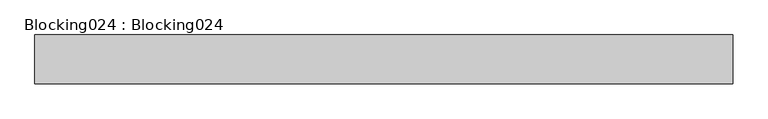
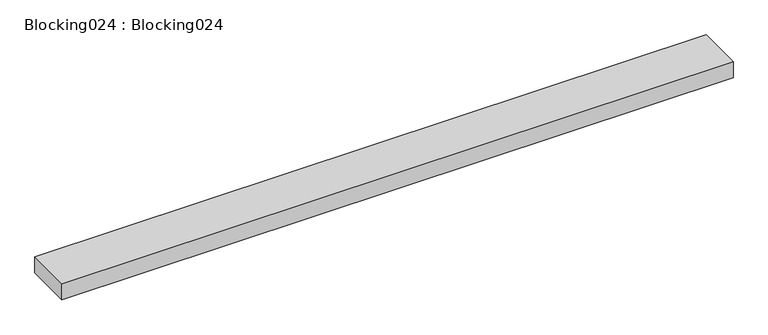
"""IFC4 building model written with IfcOpenShell, lengths in millimetres: proxy geometry, Blocking024 : Blocking024."""

from ifc_helpers import new_model, si_unit, frame, origin, place, context, project, spatial, polyline, outline, extrude, source, transform, mapped, element, save


def blocking024_blocking024_03ddc5ce(model_context):
    return source(origin(), model_context, "Body", "SweptSolid", [
        extrude(outline(polyline([(14383.0178845, -4497.8417972), (14383.0178845, -4637.5417972), (12383.0178845, -4637.5417972), (12383.0178845, -4497.8417972), (14383.0178845, -4497.8417972)])), frame((0.0, 0.0, 36531.296), z_axis=(0.0, 0.0, 1.0), x_axis=(1.0, 0.0, 0.0)), (0.0, 0.0, 1.0), 50.8),
    ])


if __name__ == "__main__":
    model = new_model("IFC4")
    model_context = context("Model", 3, world=origin())
    ifc_project = project(units=[si_unit("LENGTHUNIT", "METRE", prefix="MILLI")], contexts=[model_context])
    site = spatial("IfcSite", under=ifc_project)
    building = spatial("IfcBuilding", under=site)
    placement = place(None, origin())
    blocking024_blocking024_shape = blocking024_blocking024_03ddc5ce(model_context)
    element("IfcBuildingElementProxy", 1, Name="Blocking024 : Blocking024", ObjectType="Blocking024 : Blocking024", at=placement, inside=building, context=model_context, shape_type="MappedRepresentation", body=[
        mapped(blocking024_blocking024_shape, transform((0.0, 0.0, 0.0), x_axis=(1.0, 0.0, 0.0), y_axis=(0.0, 1.0, 0.0), z_axis=(0.0, 0.0, 1.0))),
    ])
    save(model, "model.ifc")

# Revit data of these elements
# Type "Blocking024 : Blocking024"
#   NameOverride = "Blocking024"
# Element 1 (IfcBuildingElementProxy, "Blocking024 : Blocking024")
#   Materials on its faces: "WOOD BLOCKING AS REQUIRED"
# Materials
#   "WOOD BLOCKING AS REQUIRED": class "Unassigned", colour RGB 166 124 85, transparency 0, Cost = 0
